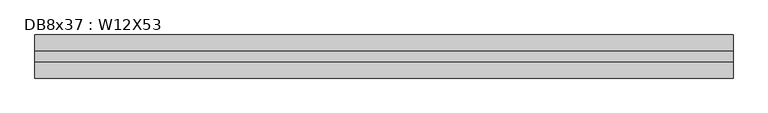
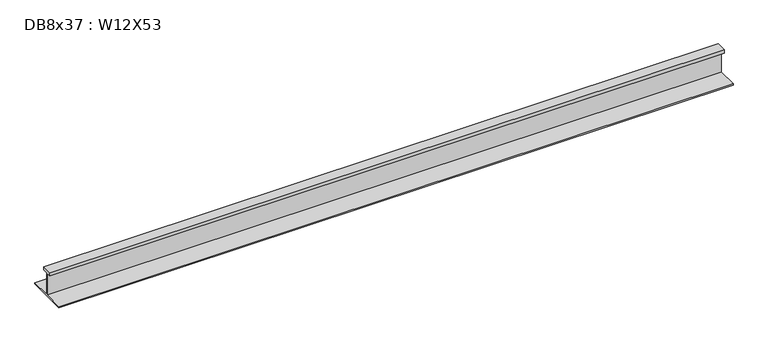
"""IFC4 building model written with IfcOpenShell, lengths in millimetres: beam geometry, DB8x37 : W12X53."""

from ifc_helpers import new_model, si_unit, frame, origin, place, context, project, spatial, polyline, outline, extrude, source, transform, mapped, element, save


def db8x37_w12x53_5ca4f80d(model_context):
    return source(origin(), model_context, "Body", "SweptSolid", [
        extrude(outline(polyline([(38.1, 145.415), (38.1, 120.015), (2.921, 120.015), (2.921, -48.4505), (152.4, -48.4505), (152.4, -58.1025), (-152.4, -58.1025), (-152.4, -48.4505), (-2.921, -48.4505), (-2.921, 120.015), (-38.1, 120.015), (-38.1, 145.415), (38.1, 145.415)])), frame((-2467.229, 0.0, 0.0), z_axis=(1.0, 0.0, 0.0), x_axis=(0.0, 1.0, 0.0)), (0.0, 0.0, 1.0), 4934.458),
    ])


if __name__ == "__main__":
    model = new_model("IFC4")
    model_context = context("Model", 3, world=origin())
    ifc_project = project(units=[si_unit("LENGTHUNIT", "METRE", prefix="MILLI")], contexts=[model_context])
    site = spatial("IfcSite", under=ifc_project)
    building = spatial("IfcBuilding", under=site)
    placement = place(None, origin())
    db8x37_w12x53_shape = db8x37_w12x53_5ca4f80d(model_context)
    element("IfcBeam", 1, ObjectType="DB8x37 : W12X53", at=placement, inside=building, context=model_context, shape_type="MappedRepresentation", body=[
        mapped(db8x37_w12x53_shape, transform((0.0, 0.0, 0.0), x_axis=(1.0, 0.0, 0.0), y_axis=(0.0, 1.0, 0.0), z_axis=(0.0, 0.0, 1.0))),
    ])
    save(model, "model.ifc")

# Revit data of these elements
# Type "DB8x37 : W12X53"
#   Assembly Code = "B10"
#   W = 53
#   Length [instance default] = 5' - 0"
#   bf = 0' - 10"
#   d = 1' - 0.1"
#   k = 0' - 1 3/8"
#   k2 = 0' - 0.8"
#   tf = 0' - 0.575"
#   tw = 0' - 0.345"
#   A = 0.108333 SF
#   Structural Material [instance default] = Steel ASTM A992
# Element 1 (IfcBeam, "DB8x37 : W12X53")
#   Materials on its faces: "Steel ASTM A992"
# Materials
#   "Steel ASTM A992": class "Metal", colour RGB 199 199 199, transparency 0, Description = "Structural steel 50ksi", Cost = 0
